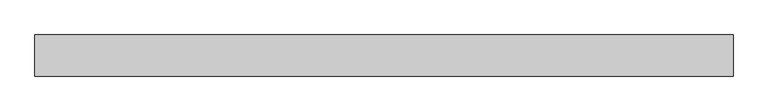
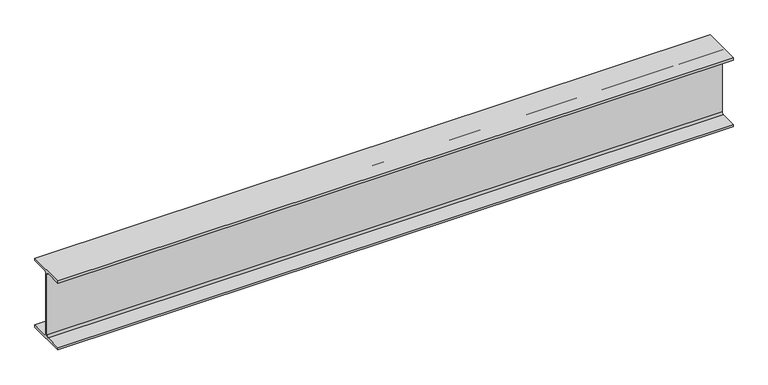
"""IFC4 building model written with IfcOpenShell, lengths in millimetres: beam geometry, Old_Steel Beam_H-KSD3502 : H_SB_ASB_H-200×200x8x12."""

from ifc_helpers import new_model, si_unit, point, frame, frame_2d, origin, place, context, project, spatial, polyline, circle_curve, trimmed, segment, composite_curve, outline, extrude, source, transform, mapped, element, save


def beam_da187b0d(model_context):
    return source(origin(), model_context, "Body", "SweptSolid", [
        extrude(outline(composite_curve([segment(polyline([(82.5, -141.5), (82.5, -151.7), (-82.5, -151.7), (-82.5, -141.5), (-11.9, -141.5)]), True, "CONTINUOUS"), segment(trimmed(circle_curve(frame_2d((-11.9, -132.6)), 8.9), [point((-11.9, -141.5))], [point((-3.0, -132.6))], True, "CARTESIAN"), True, "CONTINUOUS"), segment(polyline([(-3.0, -132.6), (-3.0, 132.6)]), True, "CONTINUOUS"), segment(trimmed(circle_curve(frame_2d((-11.9, 132.6)), 8.9), [point((-3.0, 132.6))], [point((-11.9, 141.5))], True, "CARTESIAN"), True, "CONTINUOUS"), segment(polyline([(-11.9, 141.5), (-82.5, 141.5), (-82.5, 151.7), (82.5, 151.7), (82.5, 141.5), (11.9, 141.5)]), True, "CONTINUOUS"), segment(trimmed(circle_curve(frame_2d((11.9, 132.6)), 8.9), [point((11.9, 141.5))], [point((3.0, 132.6))], True, "CARTESIAN"), True, "CONTINUOUS"), segment(polyline([(3.0, 132.6), (3.0, -132.6)]), True, "CONTINUOUS"), segment(trimmed(circle_curve(frame_2d((11.9, -132.6)), 8.9), [point((3.0, -132.6))], [point((11.9, -141.5))], True, "CARTESIAN"), True, "CONTINUOUS"), segment(polyline([(11.9, -141.5), (82.5, -141.5)]), True, "CONTINUOUS")], self_intersect=False)), frame((-1369.9070509, 0.0, 0.0), z_axis=(1.0, 0.0, 0.0), x_axis=(0.0, 1.0, 0.0)), (0.0, 0.0, 1.0), 2801.3094314),
    ])


if __name__ == "__main__":
    model = new_model("IFC4")
    model_context = context("Model", 3, world=origin())
    ifc_project = project(units=[si_unit("LENGTHUNIT", "METRE", prefix="MILLI")], contexts=[model_context])
    site = spatial("IfcSite", under=ifc_project)
    building = spatial("IfcBuilding", under=site)
    placement = place(None, origin())
    beam_shape = beam_da187b0d(model_context)
    element("IfcBeam", 1, ObjectType="Old_Steel Beam_H-KSD3502 : H_SB_ASB_H-200×200x8x12", at=placement, inside=building, context=model_context, shape_type="MappedRepresentation", body=[
        mapped(beam_shape, transform((0.0, 0.0, 0.0), x_axis=(1.0, 0.0, 0.0), y_axis=(0.0, 1.0, 0.0), z_axis=(0.0, 0.0, 1.0))),
    ])
    save(model, "model.ifc")

# Revit data of these elements
# Type "Old_Steel Beam_H-KSD3502 : H_SB_ASB_H-200×200x8x12"
#   Width = 20.0 cm
#   Web Thickness = 0.8 cm
#   Web Fillet = 1.3 cm
#   Warping Constant = 141376.0 cm⁶
#   Torsional Moment of Inertia = 26.2485 cm⁴
#   Torsional Modulus = 1.0 cm³
#   Section Area = 63.53 cm²
#   Plastic Modulus weak axis = 244.0 cm³
#   Plastic Modulus strong axis = 525.0 cm³
#   Perimeter = 1.16 m²/m
#   Nominal Weight = 49.90 kgf/m
#   Moment of Inertia weak axis = 1600.00 cm⁴
#   Moment of Inertia strong axis = 4720.00 cm⁴
#   Height = 20.0 cm
#   Flange Thickness = 1.2 cm
#   Elastic Modulus weak axis = 160.0 cm³
#   Elastic Modulus strong axis = 472.0 cm³
#   Centroid Vertical = 10.0 cm
#   Centroid Horizontal = 10.0 cm
#   Length [instance default] = 1.5240 m
#   Structural Material [instance default] = Steel, 45-345
#   Assembly Code = ""
# Element 1 (IfcBeam, "Old_Steel Beam_H-KSD3502 : H_SB_ASB_H-200×200x8x12")
#   Structural Material = none
# Materials
#   "Steel, 45-345": class "Metal", colour RGB 189 187 185, transparency 0, Description = "Steel 345 MPa", Cost = 0
